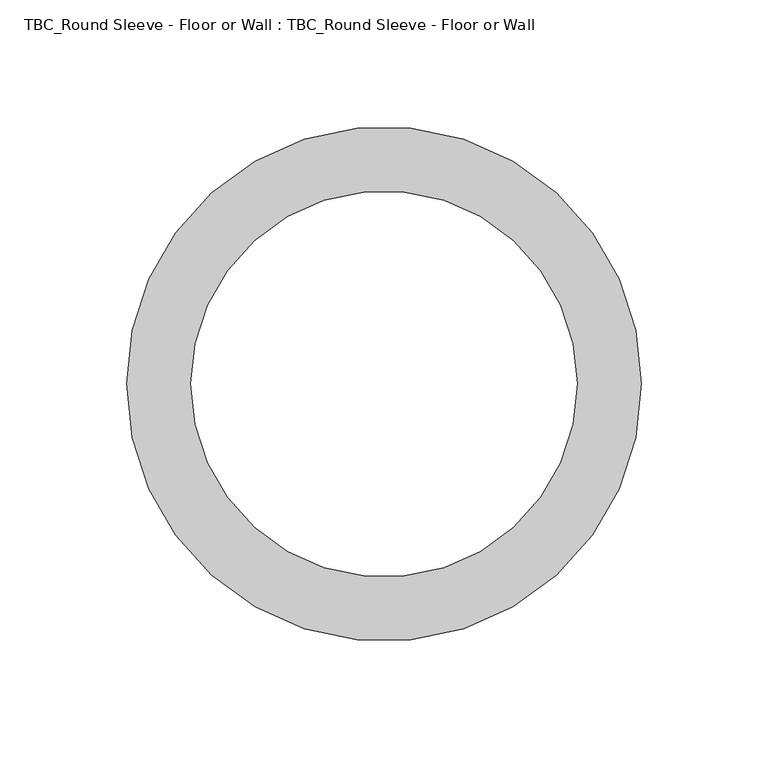
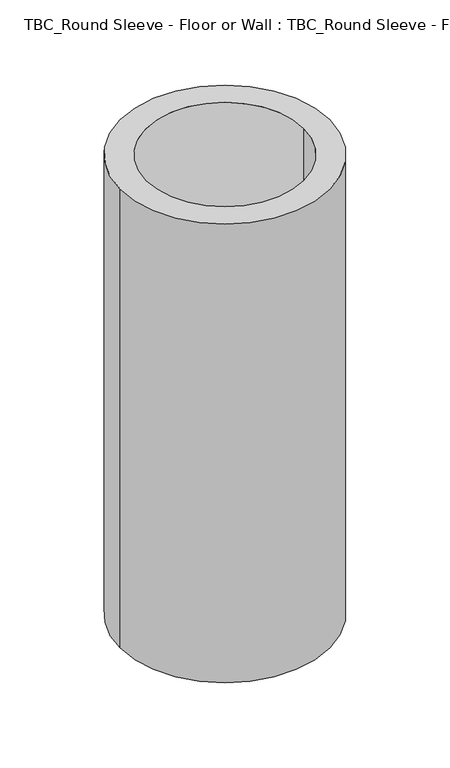
"""IFC4 building model written with IfcOpenShell, lengths in millimetres: proxy geometry, TBC_Round Sleeve - Floor or Wall : TBC_Round Sleeve - Floor or Wall."""

from ifc_helpers import new_model, si_unit, point, frame, origin, origin_2d, place, context, project, spatial, circle_curve, trimmed, segment, composite_curve, outline, extrude, source, transform, mapped, element, save


def tbc_round_sleeve_floor_or_wall_tbc_round_sleeve_floor_or_cc90379a(model_context):
    return source(origin(), model_context, "Body", "SweptSolid", [
        extrude(outline(composite_curve([segment(trimmed(circle_curve(origin_2d(), 101.6), [point((-101.6, 0.0))], [point((101.6, 0.0))], False, "CARTESIAN"), True, "CONTINUOUS"), segment(trimmed(circle_curve(origin_2d(), 101.6), [point((101.6, 0.0))], [point((-101.6, 0.0))], False, "CARTESIAN"), True, "CONTINUOUS")], self_intersect=False), holes=[composite_curve([segment(trimmed(circle_curve(origin_2d(), 76.2), [point((-76.2, 0.0))], [point((76.2, 0.0))], True, "CARTESIAN"), True, "CONTINUOUS"), segment(trimmed(circle_curve(origin_2d(), 76.2), [point((76.2, 0.0))], [point((-76.2, 0.0))], True, "CARTESIAN"), True, "CONTINUOUS")], self_intersect=False)]), frame((0.0, 0.0, -469.9), z_axis=(0.0, 0.0, 1.0), x_axis=(1.0, 0.0, 0.0)), (0.0, 0.0, 1.0), 469.9),
    ])


if __name__ == "__main__":
    model = new_model("IFC4")
    model_context = context("Model", 3, world=origin())
    ifc_project = project(units=[si_unit("LENGTHUNIT", "METRE", prefix="MILLI")], contexts=[model_context])
    site = spatial("IfcSite", under=ifc_project)
    building = spatial("IfcBuilding", under=site)
    placement = place(None, origin())
    tbc_round_sleeve_floor_or_wall_tbc_round_sleeve_floor_or_shape = tbc_round_sleeve_floor_or_wall_tbc_round_sleeve_floor_or_cc90379a(model_context)
    element("IfcBuildingElementProxy", 1, Name="TBC_Round Sleeve - Floor or Wall : TBC_Round Sleeve - Floor or Wall", ObjectType="TBC_Round Sleeve - Floor or Wall : TBC_Round Sleeve - Floor or Wall", at=placement, inside=building, context=model_context, shape_type="MappedRepresentation", body=[
        mapped(tbc_round_sleeve_floor_or_wall_tbc_round_sleeve_floor_or_shape, transform((0.0, 0.0, 0.0), x_axis=(1.0, 0.0, 0.0), y_axis=(0.0, 1.0, 0.0), z_axis=(0.0, 0.0, 1.0))),
    ])
    save(model, "model.ifc")

# Revit data of these elements
# Type "TBC_Round Sleeve - Floor or Wall : TBC_Round Sleeve - Floor or Wall"
#   Tag Dimension [instance default] = ""
#   MEP Type [instance default] = ""
#   MEP Element [instance default] = ""
#   MEP Category [instance default] = ""
#   Host Element Type [instance default] = ""
#   Host Element Id [instance default] = ""
#   Host Element Category [instance default] = ""
#   Control Line Y [instance default] = ""
#   Control Line X [instance default] = ""
#   Sleeve Radius [instance default] = 1' - 0"
#   Sleeve Edge [instance default] = 1' - 2"
#   Sleeve Depth [instance default] = 3' - 0"
#   Distance Y [instance default] = 0' - 0"
#   Distance X [instance default] = 0' - 0"
#   Default Elevation = 0
# Element 1 (IfcBuildingElementProxy, "TBC_Round Sleeve - Floor or Wall : TBC_Round Sleeve - Floor or Wall")
#   Tag Dimension = "8\"ø"
#   MEP Type = "PLG-ST"
#   MEP Element = "829932"
#   MEP Category = "Pipe"
#   Host Element Type = "Roof System A"
#   Host Element Id = "1229465"
#   Host Element Category = "Roofs"
#   Sleeve Radius = 0' - 6"
#   Sleeve Edge = 0' - 8"
#   Sleeve Depth = 1' - 6 1/2"
